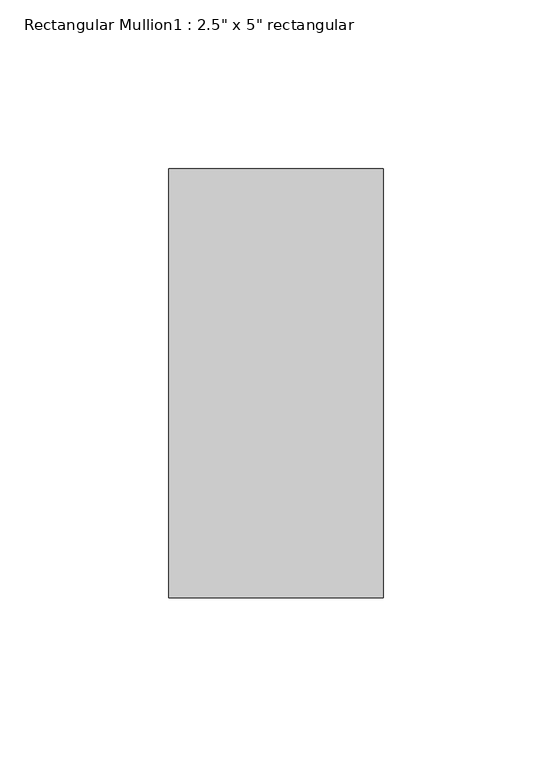
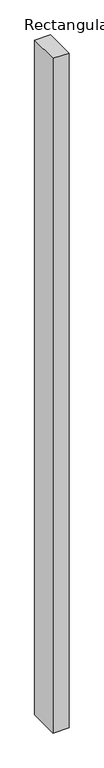
"""IFC4 building model written with IfcOpenShell, lengths in millimetres: member geometry."""

import ifcopenshell
import ifcopenshell.guid

model = None  # the IFC model being written
_history = None  # IfcOwnerHistory: only IFC2X3 demands one
_inside = {}  # id of a spatial element -> (the spatial element, [elements in it])
_under = {}  # id of a project, library or spatial element -> (it, [spatial elements below it])
_declared = {}  # id of a project -> (the project, [libraries it declares])
_typed = {}  # id of a type object -> (the type object, [elements of that type])
_made_of = {}  # id of a material, layer set ... -> (it, [elements and type objects made of it])


def new_model(schema):
    """Start an empty IFC model of exactly this schema.

    Asked for "IFC4X3", IfcOpenShell would pick the latest addendum, in which some entities
    have other attributes; the version numbers below select the first issue.
    IFC2X3 requires an IfcOwnerHistory on every rooted entity: one is made here for all.
    """
    global model, _history
    if schema == "IFC4X3":
        model = ifcopenshell.file(schema_version=(4, 3, 0, 0))
    else:
        model = ifcopenshell.file(schema=schema)
    _inside.clear()
    _under.clear()
    _declared.clear()
    _typed.clear()
    _made_of.clear()
    _history = None
    if model.schema == "IFC2X3":
        org = make("IfcOrganization", Name="unknown")
        user = make(
            "IfcPersonAndOrganization",
            ThePerson=make("IfcPerson", FamilyName="unknown"),
            TheOrganization=org,
        )
        app = make(
            "IfcApplication",
            ApplicationDeveloper=org,
            Version="unknown",
            ApplicationFullName="unknown",
            ApplicationIdentifier="unknown",
        )
        _history = make(
            "IfcOwnerHistory",
            OwningUser=user,
            OwningApplication=app,
            ChangeAction="ADDED",
            CreationDate=0,
        )
    return model


def make(cls, **values):
    """One entity of the class cls with the attributes given. An attribute that is None is left unset."""
    return model.create_entity(
        cls, **{name: value for name, value in values.items() if value is not None}
    )


def rooted(cls, **values):
    """An entity with a GlobalId (a new one), such as an element, a storey or a relation."""
    return make(cls, GlobalId=ifcopenshell.guid.new(), OwnerHistory=_history, **values)


def si_unit(unit_type, name, prefix=None):
    """IfcSIUnit, for example si_unit("LENGTHUNIT", "METRE", prefix="MILLI")."""
    return make("IfcSIUnit", UnitType=unit_type, Prefix=prefix, Name=name)


def assignment(units):
    """IfcUnitAssignment: the units of a project."""
    return None if units is None else make("IfcUnitAssignment", Units=units)


def point(xyz):
    """IfcCartesianPoint."""
    return None if xyz is None else make("IfcCartesianPoint", Coordinates=xyz)


def direction(xyz):
    """IfcDirection."""
    return None if xyz is None else make("IfcDirection", DirectionRatios=xyz)


def frame(location, z_axis=None, x_axis=None):
    """IfcAxis2Placement3D, a coordinate frame: its origin and axes. An axis left out is left unset."""
    return make(
        "IfcAxis2Placement3D",
        Location=point(location),
        Axis=direction(z_axis),
        RefDirection=direction(x_axis),
    )


def origin():
    """The frame at (0, 0, 0) with its axes left unset."""
    return frame((0.0, 0.0, 0.0))


def place(relative_to, where):
    """IfcLocalPlacement: puts the frame where relative to a parent placement (None: the world)."""
    return make(
        "IfcLocalPlacement", PlacementRelTo=relative_to, RelativePlacement=where
    )


def context(
    kind, dimensions, precision=None, world=None, true_north=None, identifier=None
):
    """IfcGeometricRepresentationContext, for example the 3D "Model" context."""
    return make(
        "IfcGeometricRepresentationContext",
        ContextIdentifier=identifier,
        ContextType=kind,
        CoordinateSpaceDimension=dimensions,
        Precision=precision,
        WorldCoordinateSystem=world,
        TrueNorth=true_north,
    )


def project(units=None, contexts=None):
    """IfcProject with its units and contexts."""
    return rooted(
        "IfcProject",
        Name="project",
        RepresentationContexts=contexts,
        UnitsInContext=assignment(units),
    )


def spatial(cls, under=None, at=None, **own):
    """A site, building, storey or space (cls), placed at a placement, below another one or the project."""
    s = rooted(cls, ObjectPlacement=at, **own)
    if under is not None:
        _under.setdefault(under.id(), (under, []))[1].append(s)
    return s


def polyline(points):
    """IfcPolyline through the points."""
    return make("IfcPolyline", Points=[point(p) for p in points])


def outline(outer, holes=None, kind="AREA"):
    """IfcArbitraryClosedProfileDef: a profile drawn as a closed curve; with holes, ...WithVoids."""
    if holes is None:
        return make("IfcArbitraryClosedProfileDef", ProfileType=kind, OuterCurve=outer)
    return make(
        "IfcArbitraryProfileDefWithVoids",
        ProfileType=kind,
        OuterCurve=outer,
        InnerCurves=holes,
    )


def extrude(swept, where, along, depth):
    """IfcExtrudedAreaSolid: the profile swept, set in the frame where, extruded along a direction by depth."""
    return make(
        "IfcExtrudedAreaSolid",
        SweptArea=swept,
        Position=where,
        ExtrudedDirection=direction(along),
        Depth=depth,
    )


def shape(context_of_items, identifier, shape_type, items):
    """IfcShapeRepresentation: the items that make up one representation, for example the "Body"."""
    return make(
        "IfcShapeRepresentation",
        ContextOfItems=context_of_items,
        RepresentationIdentifier=identifier,
        RepresentationType=shape_type,
        Items=items,
    )


def source(mapping_origin, context_of_items, identifier, shape_type, items):
    """IfcRepresentationMap: a shape defined once, which mapped items show again and again."""
    return make(
        "IfcRepresentationMap",
        MappingOrigin=mapping_origin,
        MappedRepresentation=shape(context_of_items, identifier, shape_type, items),
    )


def transform(
    local_origin,
    x_axis=None,
    y_axis=None,
    z_axis=None,
    scale=None,
    scale2=None,
    scale3=None,
    uniform=True,
):
    """IfcCartesianTransformationOperator3D, or its non-uniform kind. x_axis, y_axis, z_axis: its Axis1, 2, 3."""
    if uniform:
        return make(
            "IfcCartesianTransformationOperator3D",
            Axis1=direction(x_axis),
            Axis2=direction(y_axis),
            LocalOrigin=point(local_origin),
            Scale=scale,
            Axis3=direction(z_axis),
        )
    return make(
        "IfcCartesianTransformationOperator3DnonUniform",
        Axis1=direction(x_axis),
        Axis2=direction(y_axis),
        LocalOrigin=point(local_origin),
        Scale=scale,
        Axis3=direction(z_axis),
        Scale2=scale2,
        Scale3=scale3,
    )


def mapped(mapping_source, mapping_target):
    """IfcMappedItem: shows the shape of a source again, moved by a transform."""
    return make(
        "IfcMappedItem", MappingSource=mapping_source, MappingTarget=mapping_target
    )


def made_of(thing, what):
    """Note that an element or type object is made of a material, layer set ...; save() writes the relation."""
    if what is not None:
        _made_of.setdefault(what.id(), (what, []))[1].append(thing)
    return thing


def element(
    cls,
    number,
    at=None,
    inside=None,
    cuts=None,
    type_object=None,
    material=None,
    context=None,
    identifier="Body",
    shape_type=None,
    held_by="IfcProductDefinitionShape",
    body=None,
    shapes=None,
    **own,
):
    """One element of the class cls, such as IfcWall. Its Tag is "e" and its number.

    at: its placement. inside: the storey or other place that contains it. cuts: it is an
    opening in that element (IfcRelVoidsElement). A single representation is given by context,
    identifier, shape_type and body (its items); several are given by shapes. held_by: the class
    of the entity that holds the representations. save() writes the other relations.
    """
    e = rooted(cls, Tag="e%d" % number, ObjectPlacement=at, **own)
    if body is not None:
        shapes = [shape(context, identifier, shape_type, body)]
    if shapes is not None:
        e.Representation = make(held_by, Representations=shapes)
    if inside is not None:
        _inside.setdefault(inside.id(), (inside, []))[1].append(e)
    if cuts is not None:
        rooted(
            "IfcRelVoidsElement", RelatingBuildingElement=cuts, RelatedOpeningElement=e
        )
    if type_object is not None:
        _typed.setdefault(type_object.id(), (type_object, []))[1].append(e)
    return made_of(e, material)


def aggregate(whole, parts):
    """IfcRelAggregates: a whole, such as a stair, and the parts it consists of."""
    return rooted("IfcRelAggregates", RelatingObject=whole, RelatedObjects=parts)


def save(model, path):
    """Write the relations noted so far, then the file.

    IfcRelAggregates (storeys below a building ...), IfcRelContainedInSpatialStructure (elements
    in a storey), IfcRelDefinesByType, IfcRelAssociatesMaterial and IfcRelDeclares: one each for
    every whole, place, type object, material and project.
    """
    for whole, parts in _under.values():
        aggregate(whole, parts)
    for where, things in _inside.values():
        rooted(
            "IfcRelContainedInSpatialStructure",
            RelatedElements=things,
            RelatingStructure=where,
        )
    for kind, things in _typed.values():
        rooted("IfcRelDefinesByType", RelatedObjects=things, RelatingType=kind)
    for what, things in _made_of.values():
        rooted("IfcRelAssociatesMaterial", RelatedObjects=things, RelatingMaterial=what)
    for by, libraries in _declared.values():
        rooted("IfcRelDeclares", RelatingContext=by, RelatedDefinitions=libraries)
    model.write(path)


def member_d1cb1681(model_context):
    return source(origin(), model_context, "Body", "SweptSolid", [
        extrude(outline(polyline([(31.75, 63.5), (31.75, -63.5), (-31.75, -63.5), (-31.75, 63.5), (31.75, 63.5)])), frame((0.0, 0.0, -2852.42), z_axis=(0.0, 0.0, 1.0), x_axis=(1.0, 0.0, 0.0)), (0.0, 0.0, 1.0), 2852.42),
    ])


if __name__ == "__main__":
    model = new_model("IFC4")
    model_context = context("Model", 3, world=origin())
    ifc_project = project(units=[si_unit("LENGTHUNIT", "METRE", prefix="MILLI")], contexts=[model_context])
    site = spatial("IfcSite", under=ifc_project)
    building = spatial("IfcBuilding", under=site)
    placement = place(None, origin())
    member_shape = member_d1cb1681(model_context)
    element("IfcMember", 1, ObjectType="Rectangular Mullion1 : 2.5\" x 5\" rectangular", at=placement, inside=building, context=model_context, shape_type="MappedRepresentation", body=[
        mapped(member_shape, transform((0.0, 0.0, 0.0), x_axis=(1.0, 0.0, 0.0), y_axis=(0.0, 1.0, 0.0), z_axis=(0.0, 0.0, 1.0))),
    ])
    save(model, "model.ifc")

# Revit data of these elements
# Type "Rectangular Mullion1 : 2.5\" x 5\" rectangular"
#   built-in parameter 1007304 = 0.416667 (stored number, unit not read)
#   built-in parameter 1007301 = 0.104167 (stored number, unit not read)
#   built-in parameter 1007300 = 0.104167 (stored number, unit not read)
# Element 1 (IfcMember, "Rectangular Mullion1 : 2.5\" x 5\" rectangular")
#   Materials on its faces: "support-frame"
# Materials
#   "support-frame": class "Unassigned", colour RGB 233 233 233, transparency 0, Cost = 0
